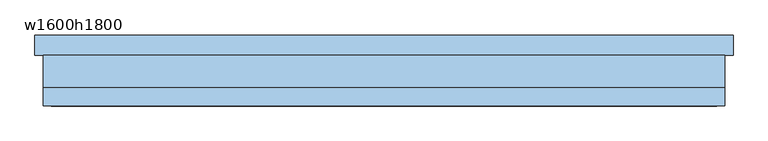
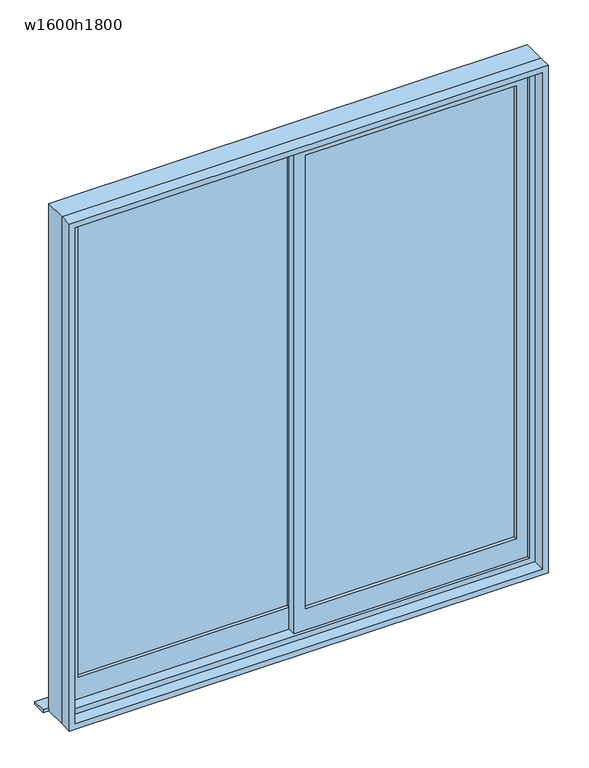
"""IFC4 building model written with IfcOpenShell, lengths in millimetres: window geometry, 引違い掃出窓_2枚 : w1600h1800."""

import ifcopenshell
import ifcopenshell.guid

model = None  # the IFC model being written
_history = None  # IfcOwnerHistory: only IFC2X3 demands one
_inside = {}  # id of a spatial element -> (the spatial element, [elements in it])
_under = {}  # id of a project, library or spatial element -> (it, [spatial elements below it])
_declared = {}  # id of a project -> (the project, [libraries it declares])
_typed = {}  # id of a type object -> (the type object, [elements of that type])
_made_of = {}  # id of a material, layer set ... -> (it, [elements and type objects made of it])


def new_model(schema):
    """Start an empty IFC model of exactly this schema.

    Asked for "IFC4X3", IfcOpenShell would pick the latest addendum, in which some entities
    have other attributes; the version numbers below select the first issue.
    IFC2X3 requires an IfcOwnerHistory on every rooted entity: one is made here for all.
    """
    global model, _history
    if schema == "IFC4X3":
        model = ifcopenshell.file(schema_version=(4, 3, 0, 0))
    else:
        model = ifcopenshell.file(schema=schema)
    _inside.clear()
    _under.clear()
    _declared.clear()
    _typed.clear()
    _made_of.clear()
    _history = None
    if model.schema == "IFC2X3":
        org = make("IfcOrganization", Name="unknown")
        user = make(
            "IfcPersonAndOrganization",
            ThePerson=make("IfcPerson", FamilyName="unknown"),
            TheOrganization=org,
        )
        app = make(
            "IfcApplication",
            ApplicationDeveloper=org,
            Version="unknown",
            ApplicationFullName="unknown",
            ApplicationIdentifier="unknown",
        )
        _history = make(
            "IfcOwnerHistory",
            OwningUser=user,
            OwningApplication=app,
            ChangeAction="ADDED",
            CreationDate=0,
        )
    return model


def make(cls, **values):
    """One entity of the class cls with the attributes given. An attribute that is None is left unset."""
    return model.create_entity(
        cls, **{name: value for name, value in values.items() if value is not None}
    )


def rooted(cls, **values):
    """An entity with a GlobalId (a new one), such as an element, a storey or a relation."""
    return make(cls, GlobalId=ifcopenshell.guid.new(), OwnerHistory=_history, **values)


def si_unit(unit_type, name, prefix=None):
    """IfcSIUnit, for example si_unit("LENGTHUNIT", "METRE", prefix="MILLI")."""
    return make("IfcSIUnit", UnitType=unit_type, Prefix=prefix, Name=name)


def assignment(units):
    """IfcUnitAssignment: the units of a project."""
    return None if units is None else make("IfcUnitAssignment", Units=units)


def point(xyz):
    """IfcCartesianPoint."""
    return None if xyz is None else make("IfcCartesianPoint", Coordinates=xyz)


def direction(xyz):
    """IfcDirection."""
    return None if xyz is None else make("IfcDirection", DirectionRatios=xyz)


def frame(location, z_axis=None, x_axis=None):
    """IfcAxis2Placement3D, a coordinate frame: its origin and axes. An axis left out is left unset."""
    return make(
        "IfcAxis2Placement3D",
        Location=point(location),
        Axis=direction(z_axis),
        RefDirection=direction(x_axis),
    )


def origin():
    """The frame at (0, 0, 0) with its axes left unset."""
    return frame((0.0, 0.0, 0.0))


def place(relative_to, where):
    """IfcLocalPlacement: puts the frame where relative to a parent placement (None: the world)."""
    return make(
        "IfcLocalPlacement", PlacementRelTo=relative_to, RelativePlacement=where
    )


def context(
    kind, dimensions, precision=None, world=None, true_north=None, identifier=None
):
    """IfcGeometricRepresentationContext, for example the 3D "Model" context."""
    return make(
        "IfcGeometricRepresentationContext",
        ContextIdentifier=identifier,
        ContextType=kind,
        CoordinateSpaceDimension=dimensions,
        Precision=precision,
        WorldCoordinateSystem=world,
        TrueNorth=true_north,
    )


def project(units=None, contexts=None):
    """IfcProject with its units and contexts."""
    return rooted(
        "IfcProject",
        Name="project",
        RepresentationContexts=contexts,
        UnitsInContext=assignment(units),
    )


def spatial(cls, under=None, at=None, **own):
    """A site, building, storey or space (cls), placed at a placement, below another one or the project."""
    s = rooted(cls, ObjectPlacement=at, **own)
    if under is not None:
        _under.setdefault(under.id(), (under, []))[1].append(s)
    return s


def polyline(points):
    """IfcPolyline through the points."""
    return make("IfcPolyline", Points=[point(p) for p in points])


def outline(outer, holes=None, kind="AREA"):
    """IfcArbitraryClosedProfileDef: a profile drawn as a closed curve; with holes, ...WithVoids."""
    if holes is None:
        return make("IfcArbitraryClosedProfileDef", ProfileType=kind, OuterCurve=outer)
    return make(
        "IfcArbitraryProfileDefWithVoids",
        ProfileType=kind,
        OuterCurve=outer,
        InnerCurves=holes,
    )


def extrude(swept, where, along, depth):
    """IfcExtrudedAreaSolid: the profile swept, set in the frame where, extruded along a direction by depth."""
    return make(
        "IfcExtrudedAreaSolid",
        SweptArea=swept,
        Position=where,
        ExtrudedDirection=direction(along),
        Depth=depth,
    )


def shape(context_of_items, identifier, shape_type, items):
    """IfcShapeRepresentation: the items that make up one representation, for example the "Body"."""
    return make(
        "IfcShapeRepresentation",
        ContextOfItems=context_of_items,
        RepresentationIdentifier=identifier,
        RepresentationType=shape_type,
        Items=items,
    )


def source(mapping_origin, context_of_items, identifier, shape_type, items):
    """IfcRepresentationMap: a shape defined once, which mapped items show again and again."""
    return make(
        "IfcRepresentationMap",
        MappingOrigin=mapping_origin,
        MappedRepresentation=shape(context_of_items, identifier, shape_type, items),
    )


def transform(
    local_origin,
    x_axis=None,
    y_axis=None,
    z_axis=None,
    scale=None,
    scale2=None,
    scale3=None,
    uniform=True,
):
    """IfcCartesianTransformationOperator3D, or its non-uniform kind. x_axis, y_axis, z_axis: its Axis1, 2, 3."""
    if uniform:
        return make(
            "IfcCartesianTransformationOperator3D",
            Axis1=direction(x_axis),
            Axis2=direction(y_axis),
            LocalOrigin=point(local_origin),
            Scale=scale,
            Axis3=direction(z_axis),
        )
    return make(
        "IfcCartesianTransformationOperator3DnonUniform",
        Axis1=direction(x_axis),
        Axis2=direction(y_axis),
        LocalOrigin=point(local_origin),
        Scale=scale,
        Axis3=direction(z_axis),
        Scale2=scale2,
        Scale3=scale3,
    )


def mapped(mapping_source, mapping_target):
    """IfcMappedItem: shows the shape of a source again, moved by a transform."""
    return make(
        "IfcMappedItem", MappingSource=mapping_source, MappingTarget=mapping_target
    )


def made_of(thing, what):
    """Note that an element or type object is made of a material, layer set ...; save() writes the relation."""
    if what is not None:
        _made_of.setdefault(what.id(), (what, []))[1].append(thing)
    return thing


def element(
    cls,
    number,
    at=None,
    inside=None,
    cuts=None,
    type_object=None,
    material=None,
    context=None,
    identifier="Body",
    shape_type=None,
    held_by="IfcProductDefinitionShape",
    body=None,
    shapes=None,
    **own,
):
    """One element of the class cls, such as IfcWall. Its Tag is "e" and its number.

    at: its placement. inside: the storey or other place that contains it. cuts: it is an
    opening in that element (IfcRelVoidsElement). A single representation is given by context,
    identifier, shape_type and body (its items); several are given by shapes. held_by: the class
    of the entity that holds the representations. save() writes the other relations.
    """
    e = rooted(cls, Tag="e%d" % number, ObjectPlacement=at, **own)
    if body is not None:
        shapes = [shape(context, identifier, shape_type, body)]
    if shapes is not None:
        e.Representation = make(held_by, Representations=shapes)
    if inside is not None:
        _inside.setdefault(inside.id(), (inside, []))[1].append(e)
    if cuts is not None:
        rooted(
            "IfcRelVoidsElement", RelatingBuildingElement=cuts, RelatedOpeningElement=e
        )
    if type_object is not None:
        _typed.setdefault(type_object.id(), (type_object, []))[1].append(e)
    return made_of(e, material)


def aggregate(whole, parts):
    """IfcRelAggregates: a whole, such as a stair, and the parts it consists of."""
    return rooted("IfcRelAggregates", RelatingObject=whole, RelatedObjects=parts)


def save(model, path):
    """Write the relations noted so far, then the file.

    IfcRelAggregates (storeys below a building ...), IfcRelContainedInSpatialStructure (elements
    in a storey), IfcRelDefinesByType, IfcRelAssociatesMaterial and IfcRelDeclares: one each for
    every whole, place, type object, material and project.
    """
    for whole, parts in _under.values():
        aggregate(whole, parts)
    for where, things in _inside.values():
        rooted(
            "IfcRelContainedInSpatialStructure",
            RelatedElements=things,
            RelatingStructure=where,
        )
    for kind, things in _typed.values():
        rooted("IfcRelDefinesByType", RelatedObjects=things, RelatingType=kind)
    for what, things in _made_of.values():
        rooted("IfcRelAssociatesMaterial", RelatedObjects=things, RelatingMaterial=what)
    for by, libraries in _declared.values():
        rooted("IfcRelDeclares", RelatingContext=by, RelatedDefinitions=libraries)
    model.write(path)


def w1600h1800_8e15063a(model_context):
    return source(origin(), model_context, "Body", "SweptSolid", [
        extrude(outline(polyline([(-20.0, 12.5), (-760.0, 12.5), (-760.0, 17.5), (-20.0, 17.5), (-20.0, 12.5)])), frame((0.0, 0.0, 280.0), z_axis=(0.0, 0.0, 1.0), x_axis=(1.0, 0.0, 0.0)), (0.0, 0.0, 1.0), 1680.0),
        extrude(outline(polyline([(760.0, -17.5), (20.0, -17.5), (20.0, -12.5), (760.0, -12.5), (760.0, -17.5)])), frame((0.0, 0.0, 280.0), z_axis=(0.0, 0.0, 1.0), x_axis=(1.0, 0.0, 0.0)), (0.0, 0.0, 1.0), 1680.0),
        extrude(outline(polyline([(2000.0, -20.0), (200.0, -20.0), (200.0, 800.0), (2000.0, 800.0), (2000.0, -20.0)]), holes=[polyline([(280.0, 760.0), (280.0, 20.0), (1960.0, 20.0), (1960.0, 760.0), (280.0, 760.0)])]), frame((0.0, -30.0, 0.0), z_axis=(0.0, 1.0, 0.0), x_axis=(0.0, 0.0, 1.0)), (0.0, 0.0, 1.0), 30.0),
        extrude(outline(polyline([(2000.0, -800.0), (200.0, -800.0), (200.0, 20.0), (2000.0, 20.0), (2000.0, -800.0)]), holes=[polyline([(280.0, -20.0), (280.0, -760.0), (1960.0, -760.0), (1960.0, -20.0), (280.0, -20.0)])]), frame((0.0, 0.0, 0.0), z_axis=(0.0, 1.0, 0.0), x_axis=(0.0, 0.0, 1.0)), (0.0, 0.0, 1.0), 30.0),
        extrude(outline(polyline([(860.0, 90.0), (860.0, 40.0), (-860.0, 40.0), (-860.0, 90.0), (860.0, 90.0)])), frame((0.0, 0.0, 160.0), z_axis=(0.0, 0.0, 1.0), x_axis=(1.0, 0.0, 0.0)), (0.0, 0.0, 1.0), 10.0),
        extrude(outline(polyline([(2040.0, 840.0), (2040.0, -840.0), (160.0, -840.0), (160.0, 840.0), (2040.0, 840.0)]), holes=[polyline([(180.0, -820.0), (2020.0, -820.0), (2020.0, 820.0), (180.0, 820.0), (180.0, -820.0)])]), frame((0.0, -85.0, 0.0), z_axis=(0.0, 1.0, 0.0), x_axis=(0.0, 0.0, 1.0)), (0.0, 0.0, 1.0), 45.0),
        extrude(outline(polyline([(2040.0, -840.0), (160.0, -840.0), (160.0, 840.0), (2040.0, 840.0), (2040.0, -840.0)]), holes=[polyline([(2000.0, 800.0), (200.0, 800.0), (200.0, -800.0), (2000.0, -800.0), (2000.0, 800.0)])]), frame((0.0, -40.0, 0.0), z_axis=(0.0, 1.0, 0.0), x_axis=(0.0, 0.0, 1.0)), (0.0, 0.0, 1.0), 80.0),
    ])


if __name__ == "__main__":
    model = new_model("IFC4")
    model_context = context("Model", 3, world=origin())
    ifc_project = project(units=[si_unit("LENGTHUNIT", "METRE", prefix="MILLI")], contexts=[model_context])
    site = spatial("IfcSite", under=ifc_project)
    building = spatial("IfcBuilding", under=site)
    placement = place(None, origin())
    w1600h1800_shape = w1600h1800_8e15063a(model_context)
    element("IfcWindow", 1, ObjectType="引違い掃出窓_2枚 : w1600h1800", at=placement, inside=building, context=model_context, shape_type="MappedRepresentation", body=[
        mapped(w1600h1800_shape, transform((0.0, 0.0, 0.0), x_axis=(1.0, 0.0, 0.0), y_axis=(0.0, 1.0, 0.0), z_axis=(0.0, 0.0, 1.0))),
    ])
    save(model, "model.ifc")

# Revit data of these elements
# Type "引違い掃出窓_2枚 : w1600h1800"
#   Construction Type Id = "GSP4R"
#   Analytic Construction = "1/8 インチ ピルキントン一重ガラス"
#   Type Mark = "67"
#   Operation = "ダブル パネル縦"
#   Keynote = "08520.R1"
#   Visual Light Transmittance = 0.9
#   Solar Heat Gain Coefficient = 0.86
#   Heat Transfer Coefficient (U) = 6.7069 W/(m²·K)
#   Height = 1800 mm
#   既定の腰高 = 200 mm
#   Width = 1600 mm
#   額縁見附 = 20 mm
#   額縁ちり = 10 mm
#   サッシ見附 = 40 mm
#   サッシの幅 = 80 mm
#   サッシ額縁 [instance default] = none
#   サッシ本体 [instance default] = none
#   サッシガラス [instance default] = ガラス - 透明
#   Manufacturer = ""
#   Wall Closure = (empty or 0)
#   Model = ""
#   Type Comments = ""
#   Assembly Code = ""
# Element 1 (IfcWindow, "引違い掃出窓_2枚 : w1600h1800")
#   Materials on its faces: "ガラス - 透明"
# Materials
#   "ガラス - 透明": class "ガラス", colour RGB 0 128 192, transparency 0.9, Cost = 0
